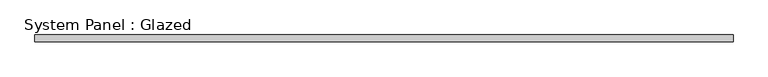
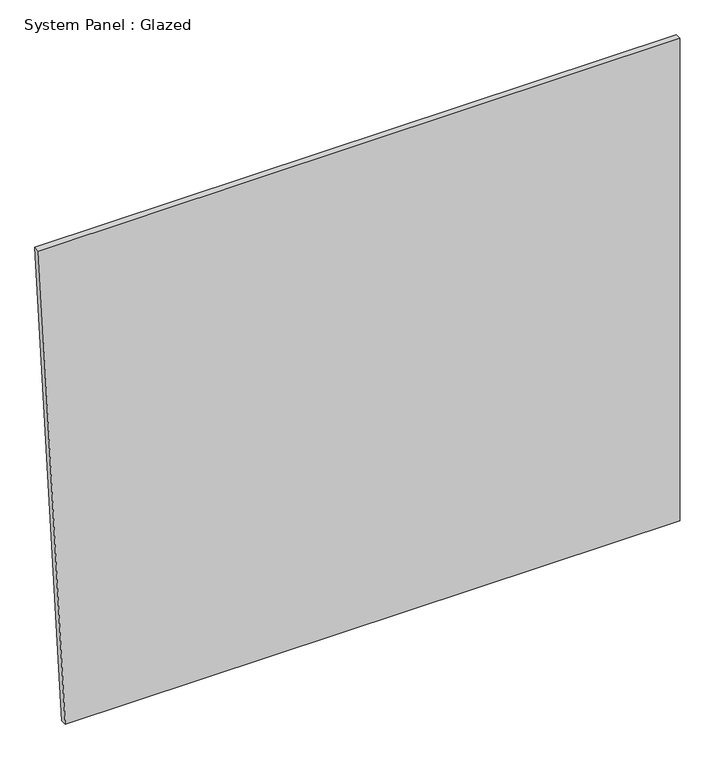
"""IFC4 building model written with IfcOpenShell, lengths in millimetres: plate geometry, System Panel : Glazed."""

from ifc_helpers import new_model, si_unit, frame, origin, place, context, project, spatial, polyline, outline, extrude, source, transform, mapped, element, save


def system_panel_glazed_02f5044a(model_context):
    return source(origin(), model_context, "Body", "SweptSolid", [
        extrude(outline(polyline([(0.0, -1204.0949696), (0.0, 1313.2352527), (2085.3785982, 1313.2352527), (2085.3785982, -1313.2352527), (0.0, -1204.0949696)])), frame((0.0, -44.45, 0.0), z_axis=(0.0, 1.0, 0.0), x_axis=(0.0, 0.0, 1.0)), (0.0, 0.0, 1.0), 25.4),
    ])


if __name__ == "__main__":
    model = new_model("IFC4")
    model_context = context("Model", 3, world=origin())
    ifc_project = project(units=[si_unit("LENGTHUNIT", "METRE", prefix="MILLI")], contexts=[model_context])
    site = spatial("IfcSite", under=ifc_project)
    building = spatial("IfcBuilding", under=site)
    placement = place(None, origin())
    system_panel_glazed_shape = system_panel_glazed_02f5044a(model_context)
    element("IfcPlate", 1, ObjectType="System Panel : Glazed", at=placement, inside=building, context=model_context, shape_type="MappedRepresentation", body=[
        mapped(system_panel_glazed_shape, transform((0.0, 0.0, 0.0), x_axis=(1.0, 0.0, 0.0), y_axis=(0.0, 1.0, 0.0), z_axis=(0.0, 0.0, 1.0))),
    ])
    save(model, "model.ifc")

# Revit data of these elements
# Type "System Panel : Glazed"
#   Construction Type Id = "GSP4R"
#   Analytic Construction = "1/8 in Pilkington single glazing"
#   Visual Light Transmittance = 0.9
#   Solar Heat Gain Coefficient = 0.86
#   Heat Transfer Coefficient (U) = 1.18115 BTU/(h·ft²·°F)
#   Define Thermal Properties by = 1
# Element 1 (IfcPlate, "System Panel : Glazed")
#   Materials on its faces: "Glass"
# Materials
#   "Glass": class "Glass", colour RGB 0 128 192, transparency 0.75, Description = "Soda Lime Glass", Cost = 0
